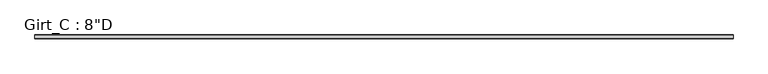
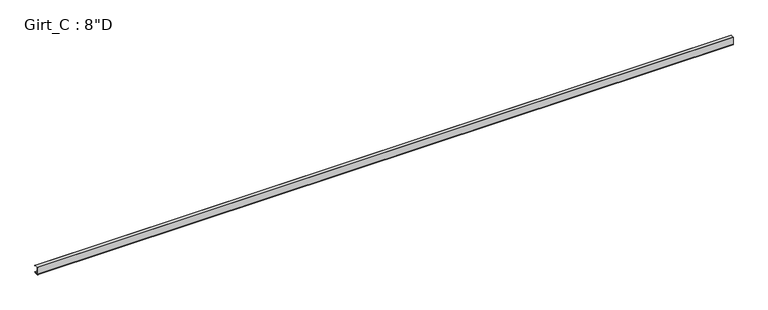
"""IFC4 building model written with IfcOpenShell, lengths in millimetres: beam geometry."""

from ifc_helpers import new_model, si_unit, point, frame, frame_2d, origin, place, context, project, spatial, polyline, circle_curve, trimmed, segment, composite_curve, outline, extrude, source, transform, mapped, element, save


def beam_e6ea6555(model_context):
    return source(origin(), model_context, "Body", "SweptSolid", [
        extrude(outline(composite_curve([segment(polyline([(87.5109375, 101.6), (99.7560415, 87.0068534), (97.6278742, 85.221109), (86.2154765, 98.821875), (3.3005807, 98.821875)]), True, "CONTINUOUS"), segment(trimmed(circle_curve(frame_2d((3.3741066, 96.8381931)), 1.9850441), [point((3.3005807, 98.821875))], [point((1.3890625, 96.8381931))], True, "CARTESIAN"), True, "CONTINUOUS"), segment(polyline([(1.3890625, 96.8381931), (1.3890625, -96.8389339)]), True, "CONTINUOUS"), segment(trimmed(circle_curve(frame_2d((3.3748024, -96.8389339)), 1.9857399), [point((1.3890625, -96.8389339))], [point((3.2694106, -98.821875))], True, "CARTESIAN"), True, "CONTINUOUS"), segment(polyline([(3.2694106, -98.821875), (86.2154765, -98.821875), (97.6510975, -85.1934327), (99.7792647, -86.979177), (87.5109375, -101.6), (3.3734375, -101.6)]), True, "CONTINUOUS"), segment(trimmed(circle_curve(frame_2d((3.3734375, -96.8375)), 4.7625), [point((3.3734375, -101.6))], [point((-1.3890625, -96.8375))], False, "CARTESIAN"), True, "CONTINUOUS"), segment(polyline([(-1.3890625, -96.8375), (-1.3890625, 96.8375)]), True, "CONTINUOUS"), segment(trimmed(circle_curve(frame_2d((3.3734375, 96.8375)), 4.7625), [point((-1.3890625, 96.8375))], [point((3.3734375, 101.6))], False, "CARTESIAN"), True, "CONTINUOUS"), segment(polyline([(3.3734375, 101.6), (87.5109375, 101.6)]), True, "CONTINUOUS")], self_intersect=False)), frame((-9004.696875, 0.0, 0.0), z_axis=(1.0, 0.0, 0.0), x_axis=(0.0, 1.0, 0.0)), (0.0, 0.0, 1.0), 17843.5),
    ])


if __name__ == "__main__":
    model = new_model("IFC4")
    model_context = context("Model", 3, world=origin())
    ifc_project = project(units=[si_unit("LENGTHUNIT", "METRE", prefix="MILLI")], contexts=[model_context])
    site = spatial("IfcSite", under=ifc_project)
    building = spatial("IfcBuilding", under=site)
    placement = place(None, origin())
    beam_shape = beam_e6ea6555(model_context)
    element("IfcBeam", 1, ObjectType="Girt_C : 8\"D", at=placement, inside=building, context=model_context, shape_type="MappedRepresentation", body=[
        mapped(beam_shape, transform((0.0, 0.0, 0.0), x_axis=(1.0, 0.0, 0.0), y_axis=(0.0, 1.0, 0.0), z_axis=(0.0, 0.0, 1.0))),
    ])
    save(model, "model.ifc")

# Revit data of these elements
# Type "Girt_C : 8\"D"
#   half leg = 0' - 1 3/4"
#   Web_Thickness = 0' - 0 7/64"
#   Length [instance default] = 10' - 0"
#   Leg_1 = 0' - 3 1/2"
#   Height = 0' - 8"
#   Structural Material [instance default] = none
# Element 1 (IfcBeam, "Girt_C : 8\"D")
#   Structural Material = CEE' SECTION (8.0x3.5C - SEE STRUCT. DWGS)
#   Materials on its faces: "CEE' SECTION (8.0x3.5C - SEE STRUCT. DWGS)"
# Materials
#   "CEE' SECTION (8.0x3.5C - SEE STRUCT. DWGS)": class "Metal", colour RGB 137 146 153, transparency 0, Description = "Steel, mill finish", Cost = 0
